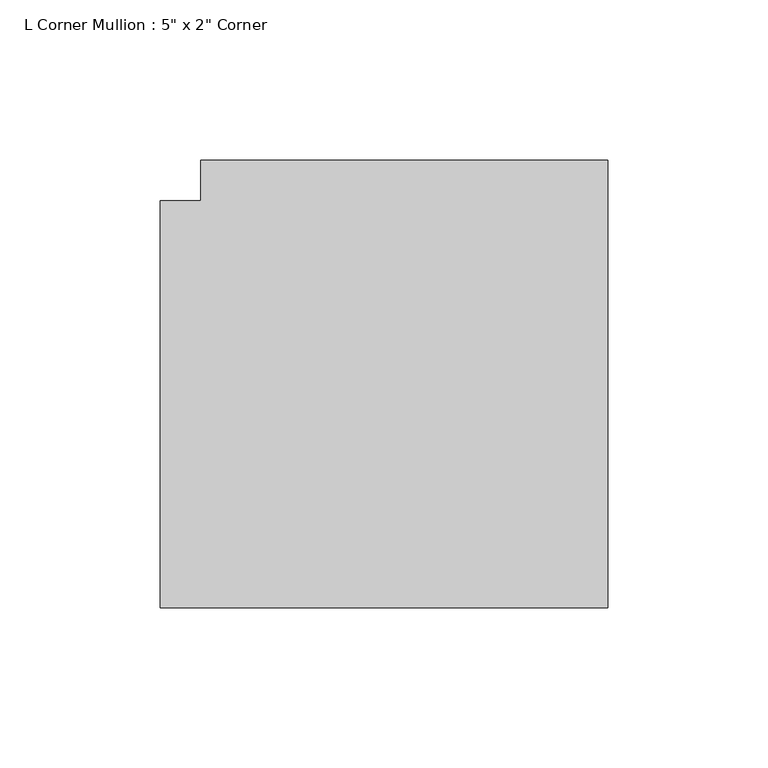
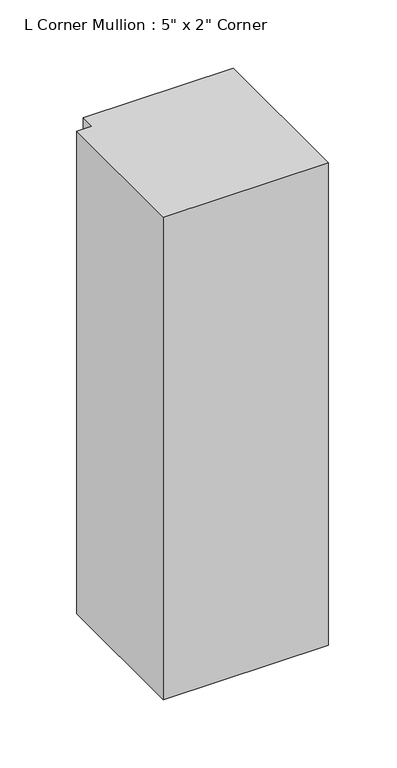
"""IFC4 building model written with IfcOpenShell, lengths in millimetres: member geometry."""

from ifc_helpers import new_model, si_unit, frame, origin, place, context, project, spatial, polyline, outline, extrude, source, transform, mapped, element, save


def member_75c5b3d2(model_context):
    return source(origin(), model_context, "Body", "SweptSolid", [
        extrude(outline(polyline([(63.5, 76.2), (63.5, -63.5), (-76.2, -63.5), (-76.2, 63.5), (-63.5, 63.5), (-63.5, 76.2), (63.5, 76.2)])), frame((0.0, 0.0, -431.8), z_axis=(0.0, 0.0, 1.0), x_axis=(1.0, 0.0, 0.0)), (0.0, 0.0, 1.0), 431.8),
    ])


if __name__ == "__main__":
    model = new_model("IFC4")
    model_context = context("Model", 3, world=origin())
    ifc_project = project(units=[si_unit("LENGTHUNIT", "METRE", prefix="MILLI")], contexts=[model_context])
    site = spatial("IfcSite", under=ifc_project)
    building = spatial("IfcBuilding", under=site)
    placement = place(None, origin())
    member_shape = member_75c5b3d2(model_context)
    element("IfcMember", 1, ObjectType="L Corner Mullion : 5\" x 2\" Corner", at=placement, inside=building, context=model_context, shape_type="MappedRepresentation", body=[
        mapped(member_shape, transform((0.0, 0.0, 0.0), x_axis=(1.0, 0.0, 0.0), y_axis=(0.0, 1.0, 0.0), z_axis=(0.0, 0.0, 1.0))),
    ])
    save(model, "model.ifc")

# Revit data of these elements
# Type "L Corner Mullion : 5\" x 2\" Corner"
#   built-in parameter 1007355 = 0.25 (stored number, unit not read)
#   built-in parameter 1007354 = 0.25 (stored number, unit not read)
#   built-in parameter 1007304 = 0.416667 (stored number, unit not read)
# Element 1 (IfcMember, "L Corner Mullion : 5\" x 2\" Corner")
#   Materials on its faces: "Metal - Aluminum"
# Materials
#   "Metal - Aluminum": class "Metal", colour RGB 109 108 108, transparency 0
